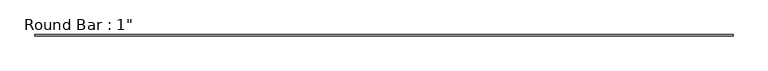
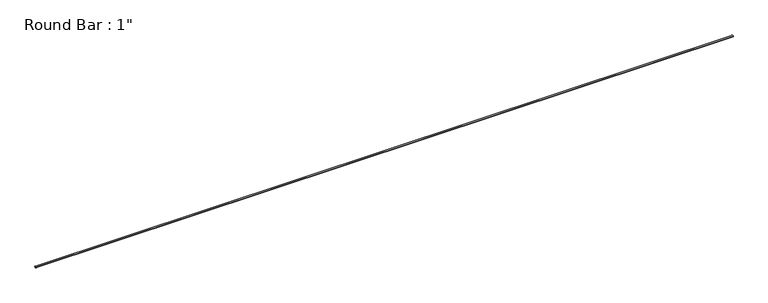
"""IFC4 building model written with IfcOpenShell, lengths in millimetres: member geometry."""

import ifcopenshell
import ifcopenshell.guid

model = None  # the IFC model being written
_history = None  # IfcOwnerHistory: only IFC2X3 demands one
_inside = {}  # id of a spatial element -> (the spatial element, [elements in it])
_under = {}  # id of a project, library or spatial element -> (it, [spatial elements below it])
_declared = {}  # id of a project -> (the project, [libraries it declares])
_typed = {}  # id of a type object -> (the type object, [elements of that type])
_made_of = {}  # id of a material, layer set ... -> (it, [elements and type objects made of it])


def new_model(schema):
    """Start an empty IFC model of exactly this schema.

    Asked for "IFC4X3", IfcOpenShell would pick the latest addendum, in which some entities
    have other attributes; the version numbers below select the first issue.
    IFC2X3 requires an IfcOwnerHistory on every rooted entity: one is made here for all.
    """
    global model, _history
    if schema == "IFC4X3":
        model = ifcopenshell.file(schema_version=(4, 3, 0, 0))
    else:
        model = ifcopenshell.file(schema=schema)
    _inside.clear()
    _under.clear()
    _declared.clear()
    _typed.clear()
    _made_of.clear()
    _history = None
    if model.schema == "IFC2X3":
        org = make("IfcOrganization", Name="unknown")
        user = make(
            "IfcPersonAndOrganization",
            ThePerson=make("IfcPerson", FamilyName="unknown"),
            TheOrganization=org,
        )
        app = make(
            "IfcApplication",
            ApplicationDeveloper=org,
            Version="unknown",
            ApplicationFullName="unknown",
            ApplicationIdentifier="unknown",
        )
        _history = make(
            "IfcOwnerHistory",
            OwningUser=user,
            OwningApplication=app,
            ChangeAction="ADDED",
            CreationDate=0,
        )
    return model


def make(cls, **values):
    """One entity of the class cls with the attributes given. An attribute that is None is left unset."""
    return model.create_entity(
        cls, **{name: value for name, value in values.items() if value is not None}
    )


def rooted(cls, **values):
    """An entity with a GlobalId (a new one), such as an element, a storey or a relation."""
    return make(cls, GlobalId=ifcopenshell.guid.new(), OwnerHistory=_history, **values)


def si_unit(unit_type, name, prefix=None):
    """IfcSIUnit, for example si_unit("LENGTHUNIT", "METRE", prefix="MILLI")."""
    return make("IfcSIUnit", UnitType=unit_type, Prefix=prefix, Name=name)


def assignment(units):
    """IfcUnitAssignment: the units of a project."""
    return None if units is None else make("IfcUnitAssignment", Units=units)


def point(xyz):
    """IfcCartesianPoint."""
    return None if xyz is None else make("IfcCartesianPoint", Coordinates=xyz)


def direction(xyz):
    """IfcDirection."""
    return None if xyz is None else make("IfcDirection", DirectionRatios=xyz)


def frame(location, z_axis=None, x_axis=None):
    """IfcAxis2Placement3D, a coordinate frame: its origin and axes. An axis left out is left unset."""
    return make(
        "IfcAxis2Placement3D",
        Location=point(location),
        Axis=direction(z_axis),
        RefDirection=direction(x_axis),
    )


def frame_2d(location, x_axis=None):
    """IfcAxis2Placement2D, a coordinate frame in the plane: its origin and x axis."""
    return make(
        "IfcAxis2Placement2D", Location=point(location), RefDirection=direction(x_axis)
    )


def origin():
    """The frame at (0, 0, 0) with its axes left unset."""
    return frame((0.0, 0.0, 0.0))


def origin_2d():
    """The frame at (0, 0) in the plane with its x axis left unset."""
    return frame_2d((0.0, 0.0))


def place(relative_to, where):
    """IfcLocalPlacement: puts the frame where relative to a parent placement (None: the world)."""
    return make(
        "IfcLocalPlacement", PlacementRelTo=relative_to, RelativePlacement=where
    )


def context(
    kind, dimensions, precision=None, world=None, true_north=None, identifier=None
):
    """IfcGeometricRepresentationContext, for example the 3D "Model" context."""
    return make(
        "IfcGeometricRepresentationContext",
        ContextIdentifier=identifier,
        ContextType=kind,
        CoordinateSpaceDimension=dimensions,
        Precision=precision,
        WorldCoordinateSystem=world,
        TrueNorth=true_north,
    )


def project(units=None, contexts=None):
    """IfcProject with its units and contexts."""
    return rooted(
        "IfcProject",
        Name="project",
        RepresentationContexts=contexts,
        UnitsInContext=assignment(units),
    )


def spatial(cls, under=None, at=None, **own):
    """A site, building, storey or space (cls), placed at a placement, below another one or the project."""
    s = rooted(cls, ObjectPlacement=at, **own)
    if under is not None:
        _under.setdefault(under.id(), (under, []))[1].append(s)
    return s


def circle_curve(where, radius):
    """IfcCircle in the frame where."""
    return make("IfcCircle", Position=where, Radius=radius)


def trimmed(basis, trim1, trim2, sense, master):
    """IfcTrimmedCurve: the piece of a basis curve between two trims."""
    return make(
        "IfcTrimmedCurve",
        BasisCurve=basis,
        Trim1=trim1,
        Trim2=trim2,
        SenseAgreement=sense,
        MasterRepresentation=master,
    )


def segment(curve, same_sense, transition):
    """IfcCompositeCurveSegment."""
    return make(
        "IfcCompositeCurveSegment",
        Transition=transition,
        SameSense=same_sense,
        ParentCurve=curve,
    )


def composite_curve(segments, self_intersect=None):
    """IfcCompositeCurve: segments joined end to end."""
    return make("IfcCompositeCurve", Segments=segments, SelfIntersect=self_intersect)


def outline(outer, holes=None, kind="AREA"):
    """IfcArbitraryClosedProfileDef: a profile drawn as a closed curve; with holes, ...WithVoids."""
    if holes is None:
        return make("IfcArbitraryClosedProfileDef", ProfileType=kind, OuterCurve=outer)
    return make(
        "IfcArbitraryProfileDefWithVoids",
        ProfileType=kind,
        OuterCurve=outer,
        InnerCurves=holes,
    )


def extrude(swept, where, along, depth):
    """IfcExtrudedAreaSolid: the profile swept, set in the frame where, extruded along a direction by depth."""
    return make(
        "IfcExtrudedAreaSolid",
        SweptArea=swept,
        Position=where,
        ExtrudedDirection=direction(along),
        Depth=depth,
    )


def shape(context_of_items, identifier, shape_type, items):
    """IfcShapeRepresentation: the items that make up one representation, for example the "Body"."""
    return make(
        "IfcShapeRepresentation",
        ContextOfItems=context_of_items,
        RepresentationIdentifier=identifier,
        RepresentationType=shape_type,
        Items=items,
    )


def source(mapping_origin, context_of_items, identifier, shape_type, items):
    """IfcRepresentationMap: a shape defined once, which mapped items show again and again."""
    return make(
        "IfcRepresentationMap",
        MappingOrigin=mapping_origin,
        MappedRepresentation=shape(context_of_items, identifier, shape_type, items),
    )


def transform(
    local_origin,
    x_axis=None,
    y_axis=None,
    z_axis=None,
    scale=None,
    scale2=None,
    scale3=None,
    uniform=True,
):
    """IfcCartesianTransformationOperator3D, or its non-uniform kind. x_axis, y_axis, z_axis: its Axis1, 2, 3."""
    if uniform:
        return make(
            "IfcCartesianTransformationOperator3D",
            Axis1=direction(x_axis),
            Axis2=direction(y_axis),
            LocalOrigin=point(local_origin),
            Scale=scale,
            Axis3=direction(z_axis),
        )
    return make(
        "IfcCartesianTransformationOperator3DnonUniform",
        Axis1=direction(x_axis),
        Axis2=direction(y_axis),
        LocalOrigin=point(local_origin),
        Scale=scale,
        Axis3=direction(z_axis),
        Scale2=scale2,
        Scale3=scale3,
    )


def mapped(mapping_source, mapping_target):
    """IfcMappedItem: shows the shape of a source again, moved by a transform."""
    return make(
        "IfcMappedItem", MappingSource=mapping_source, MappingTarget=mapping_target
    )


def made_of(thing, what):
    """Note that an element or type object is made of a material, layer set ...; save() writes the relation."""
    if what is not None:
        _made_of.setdefault(what.id(), (what, []))[1].append(thing)
    return thing


def element(
    cls,
    number,
    at=None,
    inside=None,
    cuts=None,
    type_object=None,
    material=None,
    context=None,
    identifier="Body",
    shape_type=None,
    held_by="IfcProductDefinitionShape",
    body=None,
    shapes=None,
    **own,
):
    """One element of the class cls, such as IfcWall. Its Tag is "e" and its number.

    at: its placement. inside: the storey or other place that contains it. cuts: it is an
    opening in that element (IfcRelVoidsElement). A single representation is given by context,
    identifier, shape_type and body (its items); several are given by shapes. held_by: the class
    of the entity that holds the representations. save() writes the other relations.
    """
    e = rooted(cls, Tag="e%d" % number, ObjectPlacement=at, **own)
    if body is not None:
        shapes = [shape(context, identifier, shape_type, body)]
    if shapes is not None:
        e.Representation = make(held_by, Representations=shapes)
    if inside is not None:
        _inside.setdefault(inside.id(), (inside, []))[1].append(e)
    if cuts is not None:
        rooted(
            "IfcRelVoidsElement", RelatingBuildingElement=cuts, RelatedOpeningElement=e
        )
    if type_object is not None:
        _typed.setdefault(type_object.id(), (type_object, []))[1].append(e)
    return made_of(e, material)


def aggregate(whole, parts):
    """IfcRelAggregates: a whole, such as a stair, and the parts it consists of."""
    return rooted("IfcRelAggregates", RelatingObject=whole, RelatedObjects=parts)


def save(model, path):
    """Write the relations noted so far, then the file.

    IfcRelAggregates (storeys below a building ...), IfcRelContainedInSpatialStructure (elements
    in a storey), IfcRelDefinesByType, IfcRelAssociatesMaterial and IfcRelDeclares: one each for
    every whole, place, type object, material and project.
    """
    for whole, parts in _under.values():
        aggregate(whole, parts)
    for where, things in _inside.values():
        rooted(
            "IfcRelContainedInSpatialStructure",
            RelatedElements=things,
            RelatingStructure=where,
        )
    for kind, things in _typed.values():
        rooted("IfcRelDefinesByType", RelatedObjects=things, RelatingType=kind)
    for what, things in _made_of.values():
        rooted("IfcRelAssociatesMaterial", RelatedObjects=things, RelatingMaterial=what)
    for by, libraries in _declared.values():
        rooted("IfcRelDeclares", RelatingContext=by, RelatedDefinitions=libraries)
    model.write(path)


def member_3d393e43(model_context):
    return source(origin(), model_context, "Body", "SweptSolid", [
        extrude(outline(composite_curve([segment(trimmed(circle_curve(origin_2d(), 12.7), [point((12.7, 0.0))], [point((-12.7, 0.0))], False, "CARTESIAN"), True, "CONTINUOUS"), segment(trimmed(circle_curve(origin_2d(), 12.7), [point((-12.7, 0.0))], [point((12.7, 0.0))], False, "CARTESIAN"), True, "CONTINUOUS")], self_intersect=False)), frame((-6152.7715595, 0.0, 0.0), z_axis=(1.0, 0.0, 0.0), x_axis=(0.0, 1.0, 0.0)), (0.0, 0.0, 1.0), 12305.543119),
    ])


if __name__ == "__main__":
    model = new_model("IFC4")
    model_context = context("Model", 3, world=origin())
    ifc_project = project(units=[si_unit("LENGTHUNIT", "METRE", prefix="MILLI")], contexts=[model_context])
    site = spatial("IfcSite", under=ifc_project)
    building = spatial("IfcBuilding", under=site)
    placement = place(None, origin())
    member_shape = member_3d393e43(model_context)
    element("IfcMember", 1, ObjectType="Round Bar : 1\"", at=placement, inside=building, context=model_context, shape_type="MappedRepresentation", body=[
        mapped(member_shape, transform((0.0, 0.0, 0.0), x_axis=(1.0, 0.0, 0.0), y_axis=(0.0, 1.0, 0.0), z_axis=(0.0, 0.0, 1.0))),
    ])
    save(model, "model.ifc")

# Revit data of these elements
# Type "Round Bar : 1\""
#   Assembly Code = "B10"
#   W = 0
#   Start Extension Calculation [instance default] = 10' - 0"
#   Start Extension [instance default] = -0' - 0 1/2"
#   End Extension Calculation [instance default] = 10' - 0"
#   End Extension [instance default] = -0' - 0 1/2"
#   Length [instance default] = 5' - 0"
#   d = 0' - 1"
#   A = 0 SF
#   Structural Material [instance default] = Metal - Steel - ASTM A36
# Element 1 (IfcMember, "Round Bar : 1\"")
#   Materials on its faces: "Metal - Steel - ASTM A36"
# Materials
#   "Metal - Steel - ASTM A36": class "Metal", colour RGB 199 199 199, transparency 0
